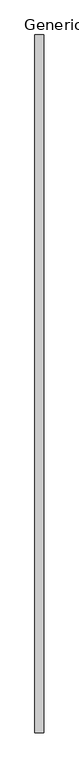
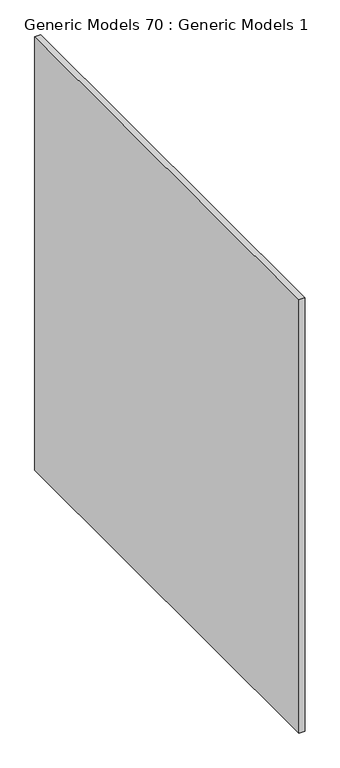
"""IFC4 building model written with IfcOpenShell, lengths in millimetres: proxy geometry, Generic Models 70 : Generic Models 1."""

from ifc_helpers import new_model, si_unit, frame, origin, place, context, project, spatial, polyline, outline, extrude, source, transform, mapped, element, save


def generic_models_70_generic_models_1_2fc778b0(model_context):
    return source(origin(), model_context, "Body", "SweptSolid", [
        extrude(outline(polyline([(51059.1296235, 0.0), (51043.2546235, 0.0), (51043.2546235, 1219.2), (51059.1296235, 1219.2), (51059.1296235, 0.0)])), frame((0.0, 0.0, 34.479891), z_axis=(0.0, 0.0, 1.0), x_axis=(1.0, 0.0, 0.0)), (0.0, 0.0, 1.0), 1219.2),
    ])


if __name__ == "__main__":
    model = new_model("IFC4")
    model_context = context("Model", 3, world=origin())
    ifc_project = project(units=[si_unit("LENGTHUNIT", "METRE", prefix="MILLI")], contexts=[model_context])
    site = spatial("IfcSite", under=ifc_project)
    building = spatial("IfcBuilding", under=site)
    placement = place(None, origin())
    generic_models_70_generic_models_1_shape = generic_models_70_generic_models_1_2fc778b0(model_context)
    element("IfcBuildingElementProxy", 1, Name="Generic Models 70 : Generic Models 1", ObjectType="Generic Models 70 : Generic Models 1", at=placement, inside=building, context=model_context, shape_type="MappedRepresentation", body=[
        mapped(generic_models_70_generic_models_1_shape, transform((0.0, 0.0, 0.0), x_axis=(1.0, 0.0, 0.0), y_axis=(0.0, 1.0, 0.0), z_axis=(0.0, 0.0, 1.0))),
    ])
    save(model, "model.ifc")

# Revit data of these elements
# Element 1 (IfcBuildingElementProxy, "Generic Models 70 : Generic Models 1")
#   Materials on its faces: "5/8\" GYP. BD"
# Materials
#   "5/8\" GYP. BD": class "Generic", colour RGB 136 135 132, transparency 0, Description = "Gypsum Wall Board", Cost = 0
